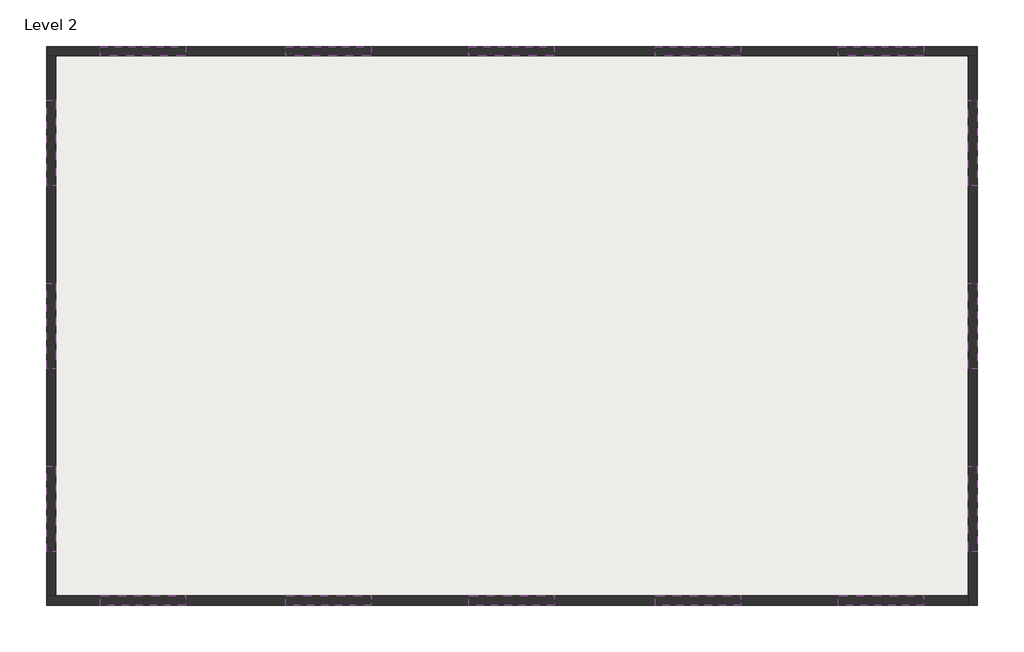
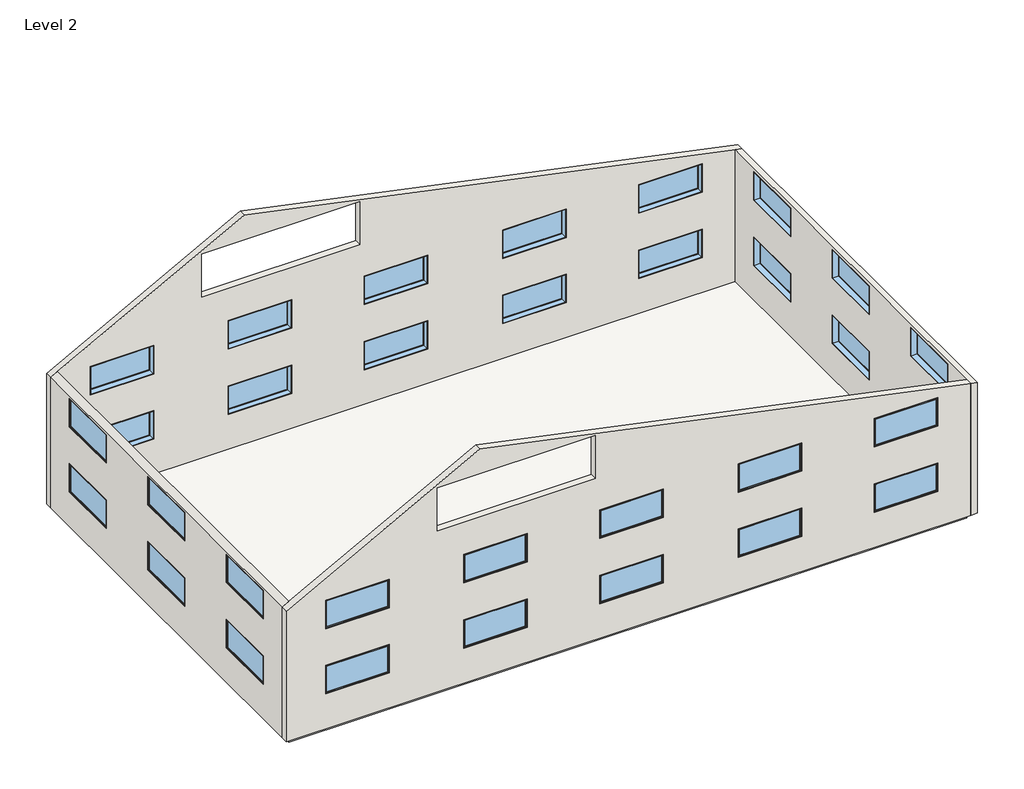
# One storey: 32 windows, 4 walls, 1 slab.
"""IFC4 building model written with IfcOpenShell, lengths in millimetres."""

import ifcopenshell
import ifcopenshell.guid

model = None  # the IFC model being written
_history = None  # IfcOwnerHistory: only IFC2X3 demands one
_inside = {}  # id of a spatial element -> (the spatial element, [elements in it])
_under = {}  # id of a project, library or spatial element -> (it, [spatial elements below it])
_declared = {}  # id of a project -> (the project, [libraries it declares])
_typed = {}  # id of a type object -> (the type object, [elements of that type])
_made_of = {}  # id of a material, layer set ... -> (it, [elements and type objects made of it])


def new_model(schema):
    """Start an empty IFC model of exactly this schema.

    Asked for "IFC4X3", IfcOpenShell would pick the latest addendum, in which some entities
    have other attributes; the version numbers below select the first issue.
    IFC2X3 requires an IfcOwnerHistory on every rooted entity: one is made here for all.
    """
    global model, _history
    if schema == "IFC4X3":
        model = ifcopenshell.file(schema_version=(4, 3, 0, 0))
    else:
        model = ifcopenshell.file(schema=schema)
    _inside.clear()
    _under.clear()
    _declared.clear()
    _typed.clear()
    _made_of.clear()
    _history = None
    if model.schema == "IFC2X3":
        org = make("IfcOrganization", Name="unknown")
        user = make(
            "IfcPersonAndOrganization",
            ThePerson=make("IfcPerson", FamilyName="unknown"),
            TheOrganization=org,
        )
        app = make(
            "IfcApplication",
            ApplicationDeveloper=org,
            Version="unknown",
            ApplicationFullName="unknown",
            ApplicationIdentifier="unknown",
        )
        _history = make(
            "IfcOwnerHistory",
            OwningUser=user,
            OwningApplication=app,
            ChangeAction="ADDED",
            CreationDate=0,
        )
    return model


def make(cls, **values):
    """One entity of the class cls with the attributes given. An attribute that is None is left unset."""
    return model.create_entity(
        cls, **{name: value for name, value in values.items() if value is not None}
    )


def rooted(cls, **values):
    """An entity with a GlobalId (a new one), such as an element, a storey or a relation."""
    return make(cls, GlobalId=ifcopenshell.guid.new(), OwnerHistory=_history, **values)


def si_unit(unit_type, name, prefix=None):
    """IfcSIUnit, for example si_unit("LENGTHUNIT", "METRE", prefix="MILLI")."""
    return make("IfcSIUnit", UnitType=unit_type, Prefix=prefix, Name=name)


def assignment(units):
    """IfcUnitAssignment: the units of a project."""
    return None if units is None else make("IfcUnitAssignment", Units=units)


def point(xyz):
    """IfcCartesianPoint."""
    return None if xyz is None else make("IfcCartesianPoint", Coordinates=xyz)


def direction(xyz):
    """IfcDirection."""
    return None if xyz is None else make("IfcDirection", DirectionRatios=xyz)


def frame(location, z_axis=None, x_axis=None):
    """IfcAxis2Placement3D, a coordinate frame: its origin and axes. An axis left out is left unset."""
    return make(
        "IfcAxis2Placement3D",
        Location=point(location),
        Axis=direction(z_axis),
        RefDirection=direction(x_axis),
    )


def origin():
    """The frame at (0, 0, 0) with its axes left unset."""
    return frame((0.0, 0.0, 0.0))


def place(relative_to, where):
    """IfcLocalPlacement: puts the frame where relative to a parent placement (None: the world)."""
    return make(
        "IfcLocalPlacement", PlacementRelTo=relative_to, RelativePlacement=where
    )


def context(
    kind, dimensions, precision=None, world=None, true_north=None, identifier=None
):
    """IfcGeometricRepresentationContext, for example the 3D "Model" context."""
    return make(
        "IfcGeometricRepresentationContext",
        ContextIdentifier=identifier,
        ContextType=kind,
        CoordinateSpaceDimension=dimensions,
        Precision=precision,
        WorldCoordinateSystem=world,
        TrueNorth=true_north,
    )


def project(units=None, contexts=None):
    """IfcProject with its units and contexts."""
    return rooted(
        "IfcProject",
        Name="project",
        RepresentationContexts=contexts,
        UnitsInContext=assignment(units),
    )


def spatial(cls, under=None, at=None, **own):
    """A site, building, storey or space (cls), placed at a placement, below another one or the project."""
    s = rooted(cls, ObjectPlacement=at, **own)
    if under is not None:
        _under.setdefault(under.id(), (under, []))[1].append(s)
    return s


def polyline(points):
    """IfcPolyline through the points."""
    return make("IfcPolyline", Points=[point(p) for p in points])


def outline(outer, holes=None, kind="AREA"):
    """IfcArbitraryClosedProfileDef: a profile drawn as a closed curve; with holes, ...WithVoids."""
    if holes is None:
        return make("IfcArbitraryClosedProfileDef", ProfileType=kind, OuterCurve=outer)
    return make(
        "IfcArbitraryProfileDefWithVoids",
        ProfileType=kind,
        OuterCurve=outer,
        InnerCurves=holes,
    )


def extrude(swept, where, along, depth):
    """IfcExtrudedAreaSolid: the profile swept, set in the frame where, extruded along a direction by depth."""
    return make(
        "IfcExtrudedAreaSolid",
        SweptArea=swept,
        Position=where,
        ExtrudedDirection=direction(along),
        Depth=depth,
    )


def faces_of(points, faces, orient=None, outer=None):
    """IfcFace entities. A face is a list of loops; a loop is a list of indices into points, from 0.

    orient and outer hold one flag for each loop. By default every Orientation is true, the
    first loop of a face is its IfcFaceOuterBound and the others are IfcFaceBound.
    """
    made = []
    for i, loops in enumerate(faces):
        bounds = []
        for j, loop in enumerate(loops):
            is_outer = j == 0 if outer is None else outer[i][j]
            bounds.append(
                make(
                    "IfcFaceOuterBound" if is_outer else "IfcFaceBound",
                    Bound=make("IfcPolyLoop", Polygon=[points[k] for k in loop]),
                    Orientation=True if orient is None else orient[i][j],
                )
            )
        made.append(make("IfcFace", Bounds=bounds))
    return made


def faceted_brep(points, faces, orient=None, outer=None, voids=None):
    """IfcFacetedBrep: a solid bounded by flat faces; with voids (closed shells), ...WithVoids."""
    shared = [point(p) for p in points]
    hull = make("IfcClosedShell", CfsFaces=faces_of(shared, faces, orient, outer))
    if voids is None:
        return make("IfcFacetedBrep", Outer=hull)
    return make(
        "IfcFacetedBrepWithVoids",
        Outer=hull,
        Voids=[
            make(cls, CfsFaces=faces_of(shared, fs, o, b)) for cls, fs, o, b in voids
        ],
    )


def shape(context_of_items, identifier, shape_type, items):
    """IfcShapeRepresentation: the items that make up one representation, for example the "Body"."""
    return make(
        "IfcShapeRepresentation",
        ContextOfItems=context_of_items,
        RepresentationIdentifier=identifier,
        RepresentationType=shape_type,
        Items=items,
    )


def source(mapping_origin, context_of_items, identifier, shape_type, items):
    """IfcRepresentationMap: a shape defined once, which mapped items show again and again."""
    return make(
        "IfcRepresentationMap",
        MappingOrigin=mapping_origin,
        MappedRepresentation=shape(context_of_items, identifier, shape_type, items),
    )


def transform(
    local_origin,
    x_axis=None,
    y_axis=None,
    z_axis=None,
    scale=None,
    scale2=None,
    scale3=None,
    uniform=True,
):
    """IfcCartesianTransformationOperator3D, or its non-uniform kind. x_axis, y_axis, z_axis: its Axis1, 2, 3."""
    if uniform:
        return make(
            "IfcCartesianTransformationOperator3D",
            Axis1=direction(x_axis),
            Axis2=direction(y_axis),
            LocalOrigin=point(local_origin),
            Scale=scale,
            Axis3=direction(z_axis),
        )
    return make(
        "IfcCartesianTransformationOperator3DnonUniform",
        Axis1=direction(x_axis),
        Axis2=direction(y_axis),
        LocalOrigin=point(local_origin),
        Scale=scale,
        Axis3=direction(z_axis),
        Scale2=scale2,
        Scale3=scale3,
    )


def mapped(mapping_source, mapping_target):
    """IfcMappedItem: shows the shape of a source again, moved by a transform."""
    return make(
        "IfcMappedItem", MappingSource=mapping_source, MappingTarget=mapping_target
    )


def made_of(thing, what):
    """Note that an element or type object is made of a material, layer set ...; save() writes the relation."""
    if what is not None:
        _made_of.setdefault(what.id(), (what, []))[1].append(thing)
    return thing


def element(
    cls,
    number,
    at=None,
    inside=None,
    cuts=None,
    type_object=None,
    material=None,
    context=None,
    identifier="Body",
    shape_type=None,
    held_by="IfcProductDefinitionShape",
    body=None,
    shapes=None,
    **own,
):
    """One element of the class cls, such as IfcWall. Its Tag is "e" and its number.

    at: its placement. inside: the storey or other place that contains it. cuts: it is an
    opening in that element (IfcRelVoidsElement). A single representation is given by context,
    identifier, shape_type and body (its items); several are given by shapes. held_by: the class
    of the entity that holds the representations. save() writes the other relations.
    """
    e = rooted(cls, Tag="e%d" % number, ObjectPlacement=at, **own)
    if body is not None:
        shapes = [shape(context, identifier, shape_type, body)]
    if shapes is not None:
        e.Representation = make(held_by, Representations=shapes)
    if inside is not None:
        _inside.setdefault(inside.id(), (inside, []))[1].append(e)
    if cuts is not None:
        rooted(
            "IfcRelVoidsElement", RelatingBuildingElement=cuts, RelatedOpeningElement=e
        )
    if type_object is not None:
        _typed.setdefault(type_object.id(), (type_object, []))[1].append(e)
    return made_of(e, material)


def aggregate(whole, parts):
    """IfcRelAggregates: a whole, such as a stair, and the parts it consists of."""
    return rooted("IfcRelAggregates", RelatingObject=whole, RelatedObjects=parts)


def save(model, path):
    """Write the relations noted so far, then the file.

    IfcRelAggregates (storeys below a building ...), IfcRelContainedInSpatialStructure (elements
    in a storey), IfcRelDefinesByType, IfcRelAssociatesMaterial and IfcRelDeclares: one each for
    every whole, place, type object, material and project.
    """
    for whole, parts in _under.values():
        aggregate(whole, parts)
    for where, things in _inside.values():
        rooted(
            "IfcRelContainedInSpatialStructure",
            RelatedElements=things,
            RelatingStructure=where,
        )
    for kind, things in _typed.values():
        rooted("IfcRelDefinesByType", RelatedObjects=things, RelatingType=kind)
    for what, things in _made_of.values():
        rooted("IfcRelAssociatesMaterial", RelatedObjects=things, RelatingMaterial=what)
    for by, libraries in _declared.values():
        rooted("IfcRelDeclares", RelatingContext=by, RelatedDefinitions=libraries)
    model.write(path)


def m_fixed_2800x_1327mm_376a1ccb(model_context):
    return source(origin(), model_context, "Body", "SweptSolid", [
        extrude(outline(polyline([(-1337.0, 130.4), (1337.0, 130.4), (1337.0, 118.4), (-1337.0, 118.4), (-1337.0, 130.4)])), frame((0.0, 0.0, 978.0), z_axis=(0.0, 0.0, 1.0), x_axis=(1.0, 0.0, 0.0)), (0.0, 0.0, 1.0), 1201.2),
        extrude(outline(polyline([(2223.2, -1381.0), (934.0, -1381.0), (934.0, 1381.0), (2223.2, 1381.0), (2223.2, -1381.0)]), holes=[polyline([(2179.2, -1337.0), (2179.2, 1337.0), (978.0, 1337.0), (978.0, -1337.0), (2179.2, -1337.0)])]), frame((0.0, 102.4, 0.0), z_axis=(0.0, 1.0, 0.0), x_axis=(0.0, 0.0, 1.0)), (0.0, 0.0, 1.0), 44.0),
        extrude(outline(polyline([(2242.2, -1400.0), (915.0, -1400.0), (915.0, 1400.0), (2242.2, 1400.0), (2242.2, -1400.0)]), holes=[polyline([(2223.2, -1381.0), (2223.2, 1381.0), (934.0, 1381.0), (934.0, -1381.0), (2223.2, -1381.0)])]), frame((0.0, 102.4, 0.0), z_axis=(0.0, 1.0, 0.0), x_axis=(0.0, 0.0, 1.0)), (0.0, 0.0, 1.0), 63.0),
        extrude(outline(polyline([(2242.2, -1400.0), (915.0, -1400.0), (915.0, 1400.0), (2242.2, 1400.0), (2242.2, -1400.0)]), holes=[polyline([(2210.2, -1368.0), (2210.2, 1368.0), (947.0, 1368.0), (947.0, -1368.0), (2210.2, -1368.0)])]), frame((0.0, -139.4, 0.0), z_axis=(0.0, 1.0, 0.0), x_axis=(0.0, 0.0, 1.0)), (0.0, 0.0, 1.0), 241.8),
    ])


def m_fixed_2800x_1327mm_95955449(model_context):
    return source(origin(), model_context, "Body", "SweptSolid", [
        extrude(outline(polyline([(-1337.0, -130.4), (-1337.0, -118.4), (1337.0, -118.4), (1337.0, -130.4), (-1337.0, -130.4)])), frame((0.0, 0.0, 978.0), z_axis=(0.0, 0.0, 1.0), x_axis=(1.0, 0.0, 0.0)), (0.0, 0.0, 1.0), 1201.2),
        extrude(outline(polyline([(2223.2, -1381.0), (934.0, -1381.0), (934.0, 1381.0), (2223.2, 1381.0), (2223.2, -1381.0)]), holes=[polyline([(2179.2, -1337.0), (2179.2, 1337.0), (978.0, 1337.0), (978.0, -1337.0), (2179.2, -1337.0)])]), frame((0.0, -146.4, 0.0), z_axis=(0.0, 1.0, 0.0), x_axis=(0.0, 0.0, 1.0)), (0.0, 0.0, 1.0), 44.0),
        extrude(outline(polyline([(2242.2, -1400.0), (915.0, -1400.0), (915.0, 1400.0), (2242.2, 1400.0), (2242.2, -1400.0)]), holes=[polyline([(2223.2, -1381.0), (2223.2, 1381.0), (934.0, 1381.0), (934.0, -1381.0), (2223.2, -1381.0)])]), frame((0.0, -165.4, 0.0), z_axis=(0.0, 1.0, 0.0), x_axis=(0.0, 0.0, 1.0)), (0.0, 0.0, 1.0), 63.0),
        extrude(outline(polyline([(2242.2, -1400.0), (915.0, -1400.0), (915.0, 1400.0), (2242.2, 1400.0), (2242.2, -1400.0)]), holes=[polyline([(2210.2, -1368.0), (2210.2, 1368.0), (947.0, 1368.0), (947.0, -1368.0), (2210.2, -1368.0)])]), frame((0.0, -102.4, 0.0), z_axis=(0.0, 1.0, 0.0), x_axis=(0.0, 0.0, 1.0)), (0.0, 0.0, 1.0), 241.8),
    ])


model = new_model("IFC4")

# Units and contexts
model_context = context("Model", 3, world=origin())
ifc_project = project(units=[si_unit("LENGTHUNIT", "METRE", prefix="MILLI")], contexts=[model_context])

# Site, building, storey
site = spatial("IfcSite", under=ifc_project)
building = spatial("IfcBuilding", under=site)
storey = spatial("IfcBuildingStorey", under=building, Name="Level 2", Elevation=3048.0)

# Slab
placement = place(None, origin())
element("IfcSlab", 1, ObjectType="Generic Floor - 304.8mm", at=placement, inside=storey, context=model_context, shape_type="SweptSolid", body=[
    extrude(outline(polyline([(31352.2035739, 12078.5990339), (31352.2035739, -5599.8009661), (1481.8035739, -5599.8009661), (1481.8035739, 12078.5990339), (31352.2035739, 12078.5990339)])), frame((0.0, 0.0, 2743.2), z_axis=(0.0, 0.0, 1.0), x_axis=(1.0, 0.0, 0.0)), (0.0, 0.0, 1.0), 304.8),
])

# Walls
element("IfcWall", 2, ObjectType="Generic - 304.8mm", at=placement, inside=storey, context=model_context, shape_type="Brep", body=[
    faceted_brep([(1177.0035739, 12078.5990339, 3048.0), (1481.8035739, 12078.5990339, 3048.0), (31352.2035739, 12078.5990339, 3048.0), (31657.0035739, 12078.5990339, 3048.0), (31657.0035739, 12078.5990339, 9144.0), (31352.2035739, 12078.5990339, 9207.5), (9711.4035739, 12078.5990339, 13716.0), (1481.8035739, 12078.5990339, 9307.2857143), (1177.0035739, 12078.5990339, 9144.0), (15004.6035739, 12078.5990339, 4643.0), (15004.6035739, 12078.5990339, 5970.2), (17804.6035739, 12078.5990339, 5970.2), (17804.6035739, 12078.5990339, 4643.0), (2929.4035739, 12078.5990339, 4666.9423249), (2929.4035739, 12078.5990339, 5994.1423249), (5729.4035739, 12078.5990339, 5994.1423249), (5729.4035739, 12078.5990339, 4666.9423249), (9004.6035739, 12078.5990339, 4666.9423249), (9004.6035739, 12078.5990339, 5994.1423249), (11804.6035739, 12078.5990339, 5994.1423249), (11804.6035739, 12078.5990339, 4666.9423249), (21104.6035739, 12078.5990339, 4666.9423249), (21104.6035739, 12078.5990339, 5994.1423249), (23904.6035739, 12078.5990339, 5994.1423249), (23904.6035739, 12078.5990339, 4666.9423249), (27104.6035739, 12078.5990339, 4666.9423249), (27104.6035739, 12078.5990339, 5994.1423249), (29904.6035739, 12078.5990339, 5994.1423249), (29904.6035739, 12078.5990339, 4666.9423249), (15004.6035739, 12078.5990339, 7691.0), (15004.6035739, 12078.5990339, 9018.2), (17804.6035739, 12078.5990339, 9018.2), (17804.6035739, 12078.5990339, 7691.0), (2929.4035739, 12078.5990339, 7714.9423249), (2929.4035739, 12078.5990339, 9042.1423249), (5729.4035739, 12078.5990339, 9042.1423249), (5729.4035739, 12078.5990339, 7714.9423249), (9004.6035739, 12078.5990339, 7714.9423249), (9004.6035739, 12078.5990339, 9042.1423249), (11804.6035739, 12078.5990339, 9042.1423249), (11804.6035739, 12078.5990339, 7714.9423249), (21104.6035739, 12078.5990339, 7714.9423249), (21104.6035739, 12078.5990339, 9042.1423249), (23904.6035739, 12078.5990339, 9042.1423249), (23904.6035739, 12078.5990339, 7714.9423249), (27104.6035739, 12078.5990339, 7714.9423249), (27104.6035739, 12078.5990339, 9042.1423249), (29904.6035739, 12078.5990339, 9042.1423249), (29904.6035739, 12078.5990339, 7714.9423249), (7845.5535739, 12078.5990339, 10559.0), (7845.5535739, 12078.5990339, 12559.0), (14813.2535739, 12078.5990339, 12559.0), (14813.2535739, 12078.5990339, 10559.0), (1177.0035739, 12383.3990339, 3048.0), (1177.0035739, 12383.3990339, 9144.0), (9711.4035739, 12383.3990339, 13716.0), (31657.0035739, 12383.3990339, 9144.0), (31657.0035739, 12383.3990339, 3048.0), (15004.6035739, 12383.3990339, 4643.0), (17804.6035739, 12383.3990339, 4643.0), (17804.6035739, 12383.3990339, 5970.2), (15004.6035739, 12383.3990339, 5970.2), (2929.4035739, 12383.3990339, 4666.9423249), (5729.4035739, 12383.3990339, 4666.9423249), (5729.4035739, 12383.3990339, 5994.1423249), (2929.4035739, 12383.3990339, 5994.1423249), (9004.6035739, 12383.3990339, 4666.9423249), (11804.6035739, 12383.3990339, 4666.9423249), (11804.6035739, 12383.3990339, 5994.1423249), (9004.6035739, 12383.3990339, 5994.1423249), (21104.6035739, 12383.3990339, 4666.9423249), (23904.6035739, 12383.3990339, 4666.9423249), (23904.6035739, 12383.3990339, 5994.1423249), (21104.6035739, 12383.3990339, 5994.1423249), (27104.6035739, 12383.3990339, 4666.9423249), (29904.6035739, 12383.3990339, 4666.9423249), (29904.6035739, 12383.3990339, 5994.1423249), (27104.6035739, 12383.3990339, 5994.1423249), (15004.6035739, 12383.3990339, 7691.0), (17804.6035739, 12383.3990339, 7691.0), (17804.6035739, 12383.3990339, 9018.2), (15004.6035739, 12383.3990339, 9018.2), (2929.4035739, 12383.3990339, 7714.9423249), (5729.4035739, 12383.3990339, 7714.9423249), (5729.4035739, 12383.3990339, 9042.1423249), (2929.4035739, 12383.3990339, 9042.1423249), (9004.6035739, 12383.3990339, 7714.9423249), (11804.6035739, 12383.3990339, 7714.9423249), (11804.6035739, 12383.3990339, 9042.1423249), (9004.6035739, 12383.3990339, 9042.1423249), (21104.6035739, 12383.3990339, 7714.9423249), (23904.6035739, 12383.3990339, 7714.9423249), (23904.6035739, 12383.3990339, 9042.1423249), (21104.6035739, 12383.3990339, 9042.1423249), (27104.6035739, 12383.3990339, 7714.9423249), (29904.6035739, 12383.3990339, 7714.9423249), (29904.6035739, 12383.3990339, 9042.1423249), (27104.6035739, 12383.3990339, 9042.1423249), (7845.5535739, 12383.3990339, 10559.0), (14813.2535739, 12383.3990339, 10559.0), (14813.2535739, 12383.3990339, 12559.0), (7845.5535739, 12383.3990339, 12559.0)], [[[0, 1, 2, 3, 4, 5, 6, 7, 8], [9, 10, 11, 12], [13, 14, 15, 16], [17, 18, 19, 20], [21, 22, 23, 24], [25, 26, 27, 28], [29, 30, 31, 32], [33, 34, 35, 36], [37, 38, 39, 40], [41, 42, 43, 44], [45, 46, 47, 48], [49, 50, 51, 52]], [[53, 54, 55, 56, 57], [58, 59, 60, 61], [62, 63, 64, 65], [66, 67, 68, 69], [70, 71, 72, 73], [74, 75, 76, 77], [78, 79, 80, 81], [82, 83, 84, 85], [86, 87, 88, 89], [90, 91, 92, 93], [94, 95, 96, 97], [98, 99, 100, 101]], [[3, 2, 1, 0, 53, 57]], [[4, 3, 57, 56]], [[0, 8, 54, 53]], [[8, 7, 6, 55, 54]], [[6, 5, 4, 56, 55]], [[10, 9, 58, 61]], [[11, 10, 61, 60]], [[12, 11, 60, 59]], [[9, 12, 59, 58]], [[14, 13, 62, 65]], [[15, 14, 65, 64]], [[16, 15, 64, 63]], [[13, 16, 63, 62]], [[18, 17, 66, 69]], [[19, 18, 69, 68]], [[20, 19, 68, 67]], [[17, 20, 67, 66]], [[22, 21, 70, 73]], [[23, 22, 73, 72]], [[24, 23, 72, 71]], [[21, 24, 71, 70]], [[26, 25, 74, 77]], [[27, 26, 77, 76]], [[28, 27, 76, 75]], [[25, 28, 75, 74]], [[30, 29, 78, 81]], [[31, 30, 81, 80]], [[32, 31, 80, 79]], [[29, 32, 79, 78]], [[34, 33, 82, 85]], [[35, 34, 85, 84]], [[36, 35, 84, 83]], [[33, 36, 83, 82]], [[38, 37, 86, 89]], [[39, 38, 89, 88]], [[40, 39, 88, 87]], [[37, 40, 87, 86]], [[42, 41, 90, 93]], [[43, 42, 93, 92]], [[44, 43, 92, 91]], [[41, 44, 91, 90]], [[46, 45, 94, 97]], [[47, 46, 97, 96]], [[48, 47, 96, 95]], [[45, 48, 95, 94]], [[50, 49, 98, 101]], [[51, 50, 101, 100]], [[52, 51, 100, 99]], [[49, 52, 99, 98]]]),
])
element("IfcWall", 3, ObjectType="Generic - 304.8mm", at=placement, inside=storey, context=model_context, shape_type="Brep", body=[
    faceted_brep([(31352.2035739, 12078.5990339, 3048.0), (31352.2035739, -5599.8009661, 3048.0), (31352.2035739, -5904.6009661, 3048.0), (31352.2035739, -5904.6009661, 9207.5), (31352.2035739, -5599.8009661, 9207.5), (31352.2035739, 12078.5990339, 9207.5), (31352.2035739, -4152.2009661, 4666.9), (31352.2035739, -1352.2009661, 4666.9), (31352.2035739, -1352.2009661, 5994.1), (31352.2035739, -4152.2009661, 5994.1), (31352.2035739, 7830.9990339, 4666.9), (31352.2035739, 10630.9990339, 4666.9), (31352.2035739, 10630.9990339, 5994.1), (31352.2035739, 7830.9990339, 5994.1), (31352.2035739, 1839.3990339, 4666.9), (31352.2035739, 4639.3990339, 4666.9), (31352.2035739, 4639.3990339, 5994.1), (31352.2035739, 1839.3990339, 5994.1), (31352.2035739, -4152.2009661, 7714.9), (31352.2035739, -1352.2009661, 7714.9), (31352.2035739, -1352.2009661, 9042.1), (31352.2035739, -4152.2009661, 9042.1), (31352.2035739, 7830.9990339, 7714.9), (31352.2035739, 10630.9990339, 7714.9), (31352.2035739, 10630.9990339, 9042.1), (31352.2035739, 7830.9990339, 9042.1), (31352.2035739, 1839.3990339, 7714.9), (31352.2035739, 4639.3990339, 7714.9), (31352.2035739, 4639.3990339, 9042.1), (31352.2035739, 1839.3990339, 9042.1), (31657.0035739, 12078.5990339, 3048.0), (31657.0035739, 12078.5990339, 9144.0), (31657.0035739, -5904.6009661, 9144.0), (31657.0035739, -5904.6009661, 3048.0), (31657.0035739, -4152.2009661, 4666.9), (31657.0035739, -4152.2009661, 5994.1), (31657.0035739, -1352.2009661, 5994.1), (31657.0035739, -1352.2009661, 4666.9), (31657.0035739, 7830.9990339, 4666.9), (31657.0035739, 7830.9990339, 5994.1), (31657.0035739, 10630.9990339, 5994.1), (31657.0035739, 10630.9990339, 4666.9), (31657.0035739, 1839.3990339, 4666.9), (31657.0035739, 1839.3990339, 5994.1), (31657.0035739, 4639.3990339, 5994.1), (31657.0035739, 4639.3990339, 4666.9), (31657.0035739, -4152.2009661, 7714.9), (31657.0035739, -4152.2009661, 9042.1), (31657.0035739, -1352.2009661, 9042.1), (31657.0035739, -1352.2009661, 7714.9), (31657.0035739, 7830.9990339, 7714.9), (31657.0035739, 7830.9990339, 9042.1), (31657.0035739, 10630.9990339, 9042.1), (31657.0035739, 10630.9990339, 7714.9), (31657.0035739, 1839.3990339, 7714.9), (31657.0035739, 1839.3990339, 9042.1), (31657.0035739, 4639.3990339, 9042.1), (31657.0035739, 4639.3990339, 7714.9)], [[[0, 1, 2, 3, 4, 5], [6, 7, 8, 9], [10, 11, 12, 13], [14, 15, 16, 17], [18, 19, 20, 21], [22, 23, 24, 25], [26, 27, 28, 29]], [[30, 31, 32, 33], [34, 35, 36, 37], [38, 39, 40, 41], [42, 43, 44, 45], [46, 47, 48, 49], [50, 51, 52, 53], [54, 55, 56, 57]], [[2, 1, 0, 30, 33]], [[0, 5, 31, 30]], [[3, 2, 33, 32]], [[35, 34, 6, 9]], [[36, 35, 9, 8]], [[37, 36, 8, 7]], [[34, 37, 7, 6]], [[39, 38, 10, 13]], [[40, 39, 13, 12]], [[41, 40, 12, 11]], [[38, 41, 11, 10]], [[43, 42, 14, 17]], [[44, 43, 17, 16]], [[45, 44, 16, 15]], [[42, 45, 15, 14]], [[47, 46, 18, 21]], [[48, 47, 21, 20]], [[49, 48, 20, 19]], [[46, 49, 19, 18]], [[51, 50, 22, 25]], [[52, 51, 25, 24]], [[53, 52, 24, 23]], [[50, 53, 23, 22]], [[55, 54, 26, 29]], [[56, 55, 29, 28]], [[57, 56, 28, 27]], [[54, 57, 27, 26]], [[5, 4, 3, 32, 31]]]),
])
element("IfcWall", 4, ObjectType="Generic - 304.8mm", at=placement, inside=storey, context=model_context, shape_type="Brep", body=[
    faceted_brep([(31352.2035739, -5599.8009661, 3048.0), (1481.8035739, -5599.8009661, 3048.0), (1177.0035739, -5599.8009661, 3048.0), (1177.0035739, -5599.8009661, 9144.0), (1481.8035739, -5599.8009661, 9307.2857143), (9711.4035739, -5599.8009661, 13716.0), (31352.2035739, -5599.8009661, 9207.5), (15004.6035739, -5599.8009661, 4643.0), (17804.6035739, -5599.8009661, 4643.0), (17804.6035739, -5599.8009661, 5970.2), (15004.6035739, -5599.8009661, 5970.2), (2929.4035739, -5599.8009661, 4666.9423249), (5729.4035739, -5599.8009661, 4666.9423249), (5729.4035739, -5599.8009661, 5994.1423249), (2929.4035739, -5599.8009661, 5994.1423249), (9004.6035739, -5599.8009661, 4666.9423249), (11804.6035739, -5599.8009661, 4666.9423249), (11804.6035739, -5599.8009661, 5994.1423249), (9004.6035739, -5599.8009661, 5994.1423249), (21104.6035739, -5599.8009661, 4666.9423249), (23904.6035739, -5599.8009661, 4666.9423249), (23904.6035739, -5599.8009661, 5994.1423249), (21104.6035739, -5599.8009661, 5994.1423249), (27104.6035739, -5599.8009661, 4666.9423249), (29904.6035739, -5599.8009661, 4666.9423249), (29904.6035739, -5599.8009661, 5994.1423249), (27104.6035739, -5599.8009661, 5994.1423249), (15004.6035739, -5599.8009661, 7691.0), (17804.6035739, -5599.8009661, 7691.0), (17804.6035739, -5599.8009661, 9018.2), (15004.6035739, -5599.8009661, 9018.2), (2929.4035739, -5599.8009661, 7714.9423249), (5729.4035739, -5599.8009661, 7714.9423249), (5729.4035739, -5599.8009661, 9042.1423249), (2929.4035739, -5599.8009661, 9042.1423249), (9004.6035739, -5599.8009661, 7714.9423249), (11804.6035739, -5599.8009661, 7714.9423249), (11804.6035739, -5599.8009661, 9042.1423249), (9004.6035739, -5599.8009661, 9042.1423249), (21104.6035739, -5599.8009661, 7714.9423249), (23904.6035739, -5599.8009661, 7714.9423249), (23904.6035739, -5599.8009661, 9042.1423249), (21104.6035739, -5599.8009661, 9042.1423249), (27104.6035739, -5599.8009661, 7714.9423249), (29904.6035739, -5599.8009661, 7714.9423249), (29904.6035739, -5599.8009661, 9042.1423249), (27104.6035739, -5599.8009661, 9042.1423249), (7845.5535739, -5599.8009661, 10559.0), (14813.2535739, -5599.8009661, 10559.0), (14813.2535739, -5599.8009661, 12559.0), (7845.5535739, -5599.8009661, 12559.0), (31352.2035739, -5904.6009661, 3048.0), (31352.2035739, -5904.6009661, 9207.5), (9711.4035739, -5904.6009661, 13716.0), (1177.0035739, -5904.6009661, 9144.0), (1177.0035739, -5904.6009661, 3048.0), (15004.6035739, -5904.6009661, 4643.0), (15004.6035739, -5904.6009661, 5970.2), (17804.6035739, -5904.6009661, 5970.2), (17804.6035739, -5904.6009661, 4643.0), (2929.4035739, -5904.6009661, 4666.9423249), (2929.4035739, -5904.6009661, 5994.1423249), (5729.4035739, -5904.6009661, 5994.1423249), (5729.4035739, -5904.6009661, 4666.9423249), (9004.6035739, -5904.6009661, 4666.9423249), (9004.6035739, -5904.6009661, 5994.1423249), (11804.6035739, -5904.6009661, 5994.1423249), (11804.6035739, -5904.6009661, 4666.9423249), (21104.6035739, -5904.6009661, 4666.9423249), (21104.6035739, -5904.6009661, 5994.1423249), (23904.6035739, -5904.6009661, 5994.1423249), (23904.6035739, -5904.6009661, 4666.9423249), (27104.6035739, -5904.6009661, 4666.9423249), (27104.6035739, -5904.6009661, 5994.1423249), (29904.6035739, -5904.6009661, 5994.1423249), (29904.6035739, -5904.6009661, 4666.9423249), (15004.6035739, -5904.6009661, 7691.0), (15004.6035739, -5904.6009661, 9018.2), (17804.6035739, -5904.6009661, 9018.2), (17804.6035739, -5904.6009661, 7691.0), (2929.4035739, -5904.6009661, 7714.9423249), (2929.4035739, -5904.6009661, 9042.1423249), (5729.4035739, -5904.6009661, 9042.1423249), (5729.4035739, -5904.6009661, 7714.9423249), (9004.6035739, -5904.6009661, 7714.9423249), (9004.6035739, -5904.6009661, 9042.1423249), (11804.6035739, -5904.6009661, 9042.1423249), (11804.6035739, -5904.6009661, 7714.9423249), (21104.6035739, -5904.6009661, 7714.9423249), (21104.6035739, -5904.6009661, 9042.1423249), (23904.6035739, -5904.6009661, 9042.1423249), (23904.6035739, -5904.6009661, 7714.9423249), (27104.6035739, -5904.6009661, 7714.9423249), (27104.6035739, -5904.6009661, 9042.1423249), (29904.6035739, -5904.6009661, 9042.1423249), (29904.6035739, -5904.6009661, 7714.9423249), (7845.5535739, -5904.6009661, 10559.0), (7845.5535739, -5904.6009661, 12559.0), (14813.2535739, -5904.6009661, 12559.0), (14813.2535739, -5904.6009661, 10559.0)], [[[0, 1, 2, 3, 4, 5, 6], [7, 8, 9, 10], [11, 12, 13, 14], [15, 16, 17, 18], [19, 20, 21, 22], [23, 24, 25, 26], [27, 28, 29, 30], [31, 32, 33, 34], [35, 36, 37, 38], [39, 40, 41, 42], [43, 44, 45, 46], [47, 48, 49, 50]], [[51, 52, 53, 54, 55], [56, 57, 58, 59], [60, 61, 62, 63], [64, 65, 66, 67], [68, 69, 70, 71], [72, 73, 74, 75], [76, 77, 78, 79], [80, 81, 82, 83], [84, 85, 86, 87], [88, 89, 90, 91], [92, 93, 94, 95], [96, 97, 98, 99]], [[2, 1, 0, 51, 55]], [[0, 6, 52, 51]], [[3, 2, 55, 54]], [[6, 5, 53, 52]], [[5, 4, 3, 54, 53]], [[57, 56, 7, 10]], [[58, 57, 10, 9]], [[59, 58, 9, 8]], [[56, 59, 8, 7]], [[61, 60, 11, 14]], [[62, 61, 14, 13]], [[63, 62, 13, 12]], [[60, 63, 12, 11]], [[65, 64, 15, 18]], [[66, 65, 18, 17]], [[67, 66, 17, 16]], [[64, 67, 16, 15]], [[69, 68, 19, 22]], [[70, 69, 22, 21]], [[71, 70, 21, 20]], [[68, 71, 20, 19]], [[73, 72, 23, 26]], [[74, 73, 26, 25]], [[75, 74, 25, 24]], [[72, 75, 24, 23]], [[77, 76, 27, 30]], [[78, 77, 30, 29]], [[79, 78, 29, 28]], [[76, 79, 28, 27]], [[81, 80, 31, 34]], [[82, 81, 34, 33]], [[83, 82, 33, 32]], [[80, 83, 32, 31]], [[85, 84, 35, 38]], [[86, 85, 38, 37]], [[87, 86, 37, 36]], [[84, 87, 36, 35]], [[89, 88, 39, 42]], [[90, 89, 42, 41]], [[91, 90, 41, 40]], [[88, 91, 40, 39]], [[93, 92, 43, 46]], [[94, 93, 46, 45]], [[95, 94, 45, 44]], [[92, 95, 44, 43]], [[97, 96, 47, 50]], [[98, 97, 50, 49]], [[99, 98, 49, 48]], [[96, 99, 48, 47]]]),
])
element("IfcWall", 5, ObjectType="Generic - 304.8mm", at=placement, inside=storey, context=model_context, shape_type="Brep", body=[
    faceted_brep([(1481.8035739, -5599.8009661, 3048.0), (1481.8035739, 12078.5990339, 3048.0), (1481.8035739, 12078.5990339, 9307.2857143), (1481.8035739, -5599.8009661, 9307.2857143), (1481.8035739, -4152.2009661, 4666.9), (1481.8035739, -4152.2009661, 5994.1), (1481.8035739, -1352.2009661, 5994.1), (1481.8035739, -1352.2009661, 4666.9), (1481.8035739, 7830.9990339, 4666.9), (1481.8035739, 7830.9990339, 5994.1), (1481.8035739, 10630.9990339, 5994.1), (1481.8035739, 10630.9990339, 4666.9), (1481.8035739, 1839.3990339, 4666.9), (1481.8035739, 1839.3990339, 5994.1), (1481.8035739, 4639.3990339, 5994.1), (1481.8035739, 4639.3990339, 4666.9), (1481.8035739, -4152.2009661, 7714.9), (1481.8035739, -4152.2009661, 9042.1), (1481.8035739, -1352.2009661, 9042.1), (1481.8035739, -1352.2009661, 7714.9), (1481.8035739, 7830.9990339, 7714.9), (1481.8035739, 7830.9990339, 9042.1), (1481.8035739, 10630.9990339, 9042.1), (1481.8035739, 10630.9990339, 7714.9), (1481.8035739, 1839.3990339, 7714.9), (1481.8035739, 1839.3990339, 9042.1), (1481.8035739, 4639.3990339, 9042.1), (1481.8035739, 4639.3990339, 7714.9), (1177.0035739, -5599.8009661, 3048.0), (1177.0035739, -5599.8009661, 9144.0), (1177.0035739, 12078.5990339, 9144.0), (1177.0035739, 12078.5990339, 3048.0), (1177.0035739, -4152.2009661, 4666.9), (1177.0035739, -1352.2009661, 4666.9), (1177.0035739, -1352.2009661, 5994.1), (1177.0035739, -4152.2009661, 5994.1), (1177.0035739, 7830.9990339, 4666.9), (1177.0035739, 10630.9990339, 4666.9), (1177.0035739, 10630.9990339, 5994.1), (1177.0035739, 7830.9990339, 5994.1), (1177.0035739, 1839.3990339, 4666.9), (1177.0035739, 4639.3990339, 4666.9), (1177.0035739, 4639.3990339, 5994.1), (1177.0035739, 1839.3990339, 5994.1), (1177.0035739, -4152.2009661, 7714.9), (1177.0035739, -1352.2009661, 7714.9), (1177.0035739, -1352.2009661, 9042.1), (1177.0035739, -4152.2009661, 9042.1), (1177.0035739, 7830.9990339, 7714.9), (1177.0035739, 10630.9990339, 7714.9), (1177.0035739, 10630.9990339, 9042.1), (1177.0035739, 7830.9990339, 9042.1), (1177.0035739, 1839.3990339, 7714.9), (1177.0035739, 4639.3990339, 7714.9), (1177.0035739, 4639.3990339, 9042.1), (1177.0035739, 1839.3990339, 9042.1)], [[[0, 1, 2, 3], [4, 5, 6, 7], [8, 9, 10, 11], [12, 13, 14, 15], [16, 17, 18, 19], [20, 21, 22, 23], [24, 25, 26, 27]], [[28, 29, 30, 31], [32, 33, 34, 35], [36, 37, 38, 39], [40, 41, 42, 43], [44, 45, 46, 47], [48, 49, 50, 51], [52, 53, 54, 55]], [[1, 0, 28, 31]], [[0, 3, 29, 28]], [[2, 1, 31, 30]], [[5, 4, 32, 35]], [[6, 5, 35, 34]], [[7, 6, 34, 33]], [[4, 7, 33, 32]], [[9, 8, 36, 39]], [[10, 9, 39, 38]], [[11, 10, 38, 37]], [[8, 11, 37, 36]], [[13, 12, 40, 43]], [[14, 13, 43, 42]], [[15, 14, 42, 41]], [[12, 15, 41, 40]], [[17, 16, 44, 47]], [[18, 17, 47, 46]], [[19, 18, 46, 45]], [[16, 19, 45, 44]], [[21, 20, 48, 51]], [[22, 21, 51, 50]], [[23, 22, 50, 49]], [[20, 23, 49, 48]], [[25, 24, 52, 55]], [[26, 25, 55, 54]], [[27, 26, 54, 53]], [[24, 27, 53, 52]], [[3, 2, 30, 29]]]),
])

# Windows
m_fixed_2800x_1327mm_shape = m_fixed_2800x_1327mm_376a1ccb(model_context)
element("IfcWindow", 6, ObjectType="M_Fixed : 2800x 1327mm", at=placement, inside=storey, context=model_context, shape_type="MappedRepresentation", body=[
    mapped(m_fixed_2800x_1327mm_shape, transform((28504.6035739, 12217.9990339, 3751.9423249), x_axis=(1.0, 0.0, 0.0), y_axis=(0.0, 1.0, 0.0), z_axis=(0.0, 0.0, 1.0))),
])
element("IfcWindow", 7, ObjectType="M_Fixed : 2800x 1327mm", at=placement, inside=storey, context=model_context, shape_type="MappedRepresentation", body=[
    mapped(m_fixed_2800x_1327mm_shape, transform((22504.6035739, 12217.9990339, 3751.9423249), x_axis=(1.0, 0.0, 0.0), y_axis=(0.0, 1.0, 0.0), z_axis=(0.0, 0.0, 1.0))),
])
element("IfcWindow", 8, ObjectType="M_Fixed : 2800x 1327mm", at=placement, inside=storey, context=model_context, shape_type="MappedRepresentation", body=[
    mapped(m_fixed_2800x_1327mm_shape, transform((10404.6035739, 12217.9990339, 3751.9423249), x_axis=(1.0, 0.0, 0.0), y_axis=(0.0, 1.0, 0.0), z_axis=(0.0, 0.0, 1.0))),
])
element("IfcWindow", 9, ObjectType="M_Fixed : 2800x 1327mm", at=placement, inside=storey, context=model_context, shape_type="MappedRepresentation", body=[
    mapped(m_fixed_2800x_1327mm_shape, transform((4329.4035739, 12217.9990339, 3751.9423249), x_axis=(1.0, 0.0, 0.0), y_axis=(0.0, 1.0, 0.0), z_axis=(0.0, 0.0, 1.0))),
])
element("IfcWindow", 10, ObjectType="M_Fixed : 2800x 1327mm", at=placement, inside=storey, context=model_context, shape_type="MappedRepresentation", body=[
    mapped(m_fixed_2800x_1327mm_shape, transform((16404.6035739, 12217.9990339, 3728.0), x_axis=(1.0, 0.0, 0.0), y_axis=(0.0, 1.0, 0.0), z_axis=(0.0, 0.0, 1.0))),
])
element("IfcWindow", 11, ObjectType="M_Fixed : 2800x 1327mm", at=placement, inside=storey, context=model_context, shape_type="MappedRepresentation", body=[
    mapped(m_fixed_2800x_1327mm_shape, transform((28504.6035739, 12217.9990339, 6799.9423249), x_axis=(1.0, 0.0, 0.0), y_axis=(0.0, 1.0, 0.0), z_axis=(0.0, 0.0, 1.0))),
])
element("IfcWindow", 12, ObjectType="M_Fixed : 2800x 1327mm", at=placement, inside=storey, context=model_context, shape_type="MappedRepresentation", body=[
    mapped(m_fixed_2800x_1327mm_shape, transform((22504.6035739, 12217.9990339, 6799.9423249), x_axis=(1.0, 0.0, 0.0), y_axis=(0.0, 1.0, 0.0), z_axis=(0.0, 0.0, 1.0))),
])
element("IfcWindow", 13, ObjectType="M_Fixed : 2800x 1327mm", at=placement, inside=storey, context=model_context, shape_type="MappedRepresentation", body=[
    mapped(m_fixed_2800x_1327mm_shape, transform((10404.6035739, 12217.9990339, 6799.9423249), x_axis=(1.0, 0.0, 0.0), y_axis=(0.0, 1.0, 0.0), z_axis=(0.0, 0.0, 1.0))),
])
element("IfcWindow", 14, ObjectType="M_Fixed : 2800x 1327mm", at=placement, inside=storey, context=model_context, shape_type="MappedRepresentation", body=[
    mapped(m_fixed_2800x_1327mm_shape, transform((4329.4035739, 12217.9990339, 6799.9423249), x_axis=(1.0, 0.0, 0.0), y_axis=(0.0, 1.0, 0.0), z_axis=(0.0, 0.0, 1.0))),
])
element("IfcWindow", 15, ObjectType="M_Fixed : 2800x 1327mm", at=placement, inside=storey, context=model_context, shape_type="MappedRepresentation", body=[
    mapped(m_fixed_2800x_1327mm_shape, transform((16404.6035739, 12217.9990339, 6776.0), x_axis=(1.0, 0.0, 0.0), y_axis=(0.0, 1.0, 0.0), z_axis=(0.0, 0.0, 1.0))),
])
element("IfcWindow", 16, ObjectType="M_Fixed : 2800x 1327mm", at=placement, inside=storey, context=model_context, shape_type="MappedRepresentation", body=[
    mapped(m_fixed_2800x_1327mm_shape, transform((1342.4035739, 3239.3990339, 3751.9), x_axis=(0.0, 1.0, 0.0), y_axis=(-1.0, 0.0, 0.0), z_axis=(0.0, 0.0, 1.0))),
])
element("IfcWindow", 17, ObjectType="M_Fixed : 2800x 1327mm", at=placement, inside=storey, context=model_context, shape_type="MappedRepresentation", body=[
    mapped(m_fixed_2800x_1327mm_shape, transform((1342.4035739, 9230.9990339, 3751.9), x_axis=(0.0, 1.0, 0.0), y_axis=(-1.0, 0.0, 0.0), z_axis=(0.0, 0.0, 1.0))),
])
element("IfcWindow", 18, ObjectType="M_Fixed : 2800x 1327mm", at=placement, inside=storey, context=model_context, shape_type="MappedRepresentation", body=[
    mapped(m_fixed_2800x_1327mm_shape, transform((1342.4035739, -2752.2009661, 3751.9), x_axis=(0.0, 1.0, 0.0), y_axis=(-1.0, 0.0, 0.0), z_axis=(0.0, 0.0, 1.0))),
])
element("IfcWindow", 19, ObjectType="M_Fixed : 2800x 1327mm", at=placement, inside=storey, context=model_context, shape_type="MappedRepresentation", body=[
    mapped(m_fixed_2800x_1327mm_shape, transform((1342.4035739, 3239.3990339, 6799.9), x_axis=(0.0, 1.0, 0.0), y_axis=(-1.0, 0.0, 0.0), z_axis=(0.0, 0.0, 1.0))),
])
element("IfcWindow", 20, ObjectType="M_Fixed : 2800x 1327mm", at=placement, inside=storey, context=model_context, shape_type="MappedRepresentation", body=[
    mapped(m_fixed_2800x_1327mm_shape, transform((1342.4035739, 9230.9990339, 6799.9), x_axis=(0.0, 1.0, 0.0), y_axis=(-1.0, 0.0, 0.0), z_axis=(0.0, 0.0, 1.0))),
])
element("IfcWindow", 21, ObjectType="M_Fixed : 2800x 1327mm", at=placement, inside=storey, context=model_context, shape_type="MappedRepresentation", body=[
    mapped(m_fixed_2800x_1327mm_shape, transform((1342.4035739, -2752.2009661, 6799.9), x_axis=(0.0, 1.0, 0.0), y_axis=(-1.0, 0.0, 0.0), z_axis=(0.0, 0.0, 1.0))),
])
m_fixed_2800x_1327mm_2_shape = m_fixed_2800x_1327mm_95955449(model_context)
element("IfcWindow", 22, ObjectType="M_Fixed : 2800x 1327mm", at=placement, inside=storey, context=model_context, shape_type="MappedRepresentation", body=[
    mapped(m_fixed_2800x_1327mm_2_shape, transform((28504.6035739, -5739.2009661, 3751.9423249), x_axis=(1.0, 0.0, 0.0), y_axis=(0.0, 1.0, 0.0), z_axis=(0.0, 0.0, 1.0))),
])
element("IfcWindow", 23, ObjectType="M_Fixed : 2800x 1327mm", at=placement, inside=storey, context=model_context, shape_type="MappedRepresentation", body=[
    mapped(m_fixed_2800x_1327mm_2_shape, transform((22504.6035739, -5739.2009661, 3751.9423249), x_axis=(1.0, 0.0, 0.0), y_axis=(0.0, 1.0, 0.0), z_axis=(0.0, 0.0, 1.0))),
])
element("IfcWindow", 24, ObjectType="M_Fixed : 2800x 1327mm", at=placement, inside=storey, context=model_context, shape_type="MappedRepresentation", body=[
    mapped(m_fixed_2800x_1327mm_2_shape, transform((10404.6035739, -5739.2009661, 3751.9423249), x_axis=(1.0, 0.0, 0.0), y_axis=(0.0, 1.0, 0.0), z_axis=(0.0, 0.0, 1.0))),
])
element("IfcWindow", 25, ObjectType="M_Fixed : 2800x 1327mm", at=placement, inside=storey, context=model_context, shape_type="MappedRepresentation", body=[
    mapped(m_fixed_2800x_1327mm_2_shape, transform((4329.4035739, -5739.2009661, 3751.9423249), x_axis=(1.0, 0.0, 0.0), y_axis=(0.0, 1.0, 0.0), z_axis=(0.0, 0.0, 1.0))),
])
element("IfcWindow", 26, ObjectType="M_Fixed : 2800x 1327mm", at=placement, inside=storey, context=model_context, shape_type="MappedRepresentation", body=[
    mapped(m_fixed_2800x_1327mm_2_shape, transform((16404.6035739, -5739.2009661, 3728.0), x_axis=(1.0, 0.0, 0.0), y_axis=(0.0, 1.0, 0.0), z_axis=(0.0, 0.0, 1.0))),
])
element("IfcWindow", 27, ObjectType="M_Fixed : 2800x 1327mm", at=placement, inside=storey, context=model_context, shape_type="MappedRepresentation", body=[
    mapped(m_fixed_2800x_1327mm_2_shape, transform((28504.6035739, -5739.2009661, 6799.9423249), x_axis=(1.0, 0.0, 0.0), y_axis=(0.0, 1.0, 0.0), z_axis=(0.0, 0.0, 1.0))),
])
element("IfcWindow", 28, ObjectType="M_Fixed : 2800x 1327mm", at=placement, inside=storey, context=model_context, shape_type="MappedRepresentation", body=[
    mapped(m_fixed_2800x_1327mm_2_shape, transform((22504.6035739, -5739.2009661, 6799.9423249), x_axis=(1.0, 0.0, 0.0), y_axis=(0.0, 1.0, 0.0), z_axis=(0.0, 0.0, 1.0))),
])
element("IfcWindow", 29, ObjectType="M_Fixed : 2800x 1327mm", at=placement, inside=storey, context=model_context, shape_type="MappedRepresentation", body=[
    mapped(m_fixed_2800x_1327mm_2_shape, transform((10404.6035739, -5739.2009661, 6799.9423249), x_axis=(1.0, 0.0, 0.0), y_axis=(0.0, 1.0, 0.0), z_axis=(0.0, 0.0, 1.0))),
])
element("IfcWindow", 30, ObjectType="M_Fixed : 2800x 1327mm", at=placement, inside=storey, context=model_context, shape_type="MappedRepresentation", body=[
    mapped(m_fixed_2800x_1327mm_2_shape, transform((4329.4035739, -5739.2009661, 6799.9423249), x_axis=(1.0, 0.0, 0.0), y_axis=(0.0, 1.0, 0.0), z_axis=(0.0, 0.0, 1.0))),
])
element("IfcWindow", 31, ObjectType="M_Fixed : 2800x 1327mm", at=placement, inside=storey, context=model_context, shape_type="MappedRepresentation", body=[
    mapped(m_fixed_2800x_1327mm_2_shape, transform((16404.6035739, -5739.2009661, 6776.0), x_axis=(1.0, 0.0, 0.0), y_axis=(0.0, 1.0, 0.0), z_axis=(0.0, 0.0, 1.0))),
])
element("IfcWindow", 32, ObjectType="M_Fixed : 2800x 1327mm", at=placement, inside=storey, context=model_context, shape_type="MappedRepresentation", body=[
    mapped(m_fixed_2800x_1327mm_2_shape, transform((31491.6035739, 3239.3990339, 3751.9), x_axis=(0.0, 1.0, 0.0), y_axis=(-1.0, 0.0, 0.0), z_axis=(0.0, 0.0, 1.0))),
])
element("IfcWindow", 33, ObjectType="M_Fixed : 2800x 1327mm", at=placement, inside=storey, context=model_context, shape_type="MappedRepresentation", body=[
    mapped(m_fixed_2800x_1327mm_2_shape, transform((31491.6035739, 9230.9990339, 3751.9), x_axis=(0.0, 1.0, 0.0), y_axis=(-1.0, 0.0, 0.0), z_axis=(0.0, 0.0, 1.0))),
])
element("IfcWindow", 34, ObjectType="M_Fixed : 2800x 1327mm", at=placement, inside=storey, context=model_context, shape_type="MappedRepresentation", body=[
    mapped(m_fixed_2800x_1327mm_2_shape, transform((31491.6035739, -2752.2009661, 3751.9), x_axis=(0.0, 1.0, 0.0), y_axis=(-1.0, 0.0, 0.0), z_axis=(0.0, 0.0, 1.0))),
])
element("IfcWindow", 35, ObjectType="M_Fixed : 2800x 1327mm", at=placement, inside=storey, context=model_context, shape_type="MappedRepresentation", body=[
    mapped(m_fixed_2800x_1327mm_2_shape, transform((31491.6035739, 3239.3990339, 6799.9), x_axis=(0.0, 1.0, 0.0), y_axis=(-1.0, 0.0, 0.0), z_axis=(0.0, 0.0, 1.0))),
])
element("IfcWindow", 36, ObjectType="M_Fixed : 2800x 1327mm", at=placement, inside=storey, context=model_context, shape_type="MappedRepresentation", body=[
    mapped(m_fixed_2800x_1327mm_2_shape, transform((31491.6035739, 9230.9990339, 6799.9), x_axis=(0.0, 1.0, 0.0), y_axis=(-1.0, 0.0, 0.0), z_axis=(0.0, 0.0, 1.0))),
])
element("IfcWindow", 37, ObjectType="M_Fixed : 2800x 1327mm", at=placement, inside=storey, context=model_context, shape_type="MappedRepresentation", body=[
    mapped(m_fixed_2800x_1327mm_2_shape, transform((31491.6035739, -2752.2009661, 6799.9), x_axis=(0.0, 1.0, 0.0), y_axis=(-1.0, 0.0, 0.0), z_axis=(0.0, 0.0, 1.0))),
])

save(model, "model.ifc")

# Revit data of these elements
# Type "Generic Floor - 304.8mm"
#   Function = 0
#   Layers, outside or top first: 304.8 mm no material (function 1)
# Type "Generic - 304.8mm"
#   Layers, outside or top first: 304.8 mm no material (function 1)
# Type "M_Fixed : 2800x 1327mm"
#   Type Mark = "46"
#   Height = 1327.2 mm
#   Default Sill Height = 915 mm
#   Width = 2800 mm
#   Window Inset = 19 mm
#   Frame Exterior Material = Sash
#   Frame Interior Material = Sash
#   Glass Pane Material = Glass
#   Sash = Sash
#   Wall Closure = (empty or 0)
# Element 1 (IfcSlab, "Generic Floor - 304.8mm")
#   Height Offset From Level = 0 mm
#   Phase Created = New Construction
#   Materials on its faces: "Default Floor"
# Elements 2, 3, 4, 5 (IfcWall, "Generic - 304.8mm")
#   Top Offset = 0 mm
#   Base Offset = 0 mm
#   wall height = 6096 mm
#   Phase Created = New Construction
#   Base Constraint = Level 2
#   Top Constraint = Roof level
#   Materials on its faces: "Default Wall"
# Element 6 (IfcWindow, "M_Fixed : 2800x 1327mm")
#   Mark = "44"
#   Phase Created = New Construction
#   Materials on its faces: "Sash", "Glass"
# Element 7 (IfcWindow, "M_Fixed : 2800x 1327mm")
#   Mark = "45"
#   Phase Created = New Construction
#   Materials on its faces: "Sash", "Glass"
# Element 8 (IfcWindow, "M_Fixed : 2800x 1327mm")
#   Mark = "46"
#   Phase Created = New Construction
#   Materials on its faces: "Sash", "Glass"
# Element 9 (IfcWindow, "M_Fixed : 2800x 1327mm")
#   Mark = "47"
#   Phase Created = New Construction
#   Materials on its faces: "Sash", "Glass"
# Element 10 (IfcWindow, "M_Fixed : 2800x 1327mm")
#   Mark = "48"
#   Phase Created = New Construction
#   Materials on its faces: "Sash", "Glass"
# Element 11 (IfcWindow, "M_Fixed : 2800x 1327mm")
#   Mark = "49"
#   Phase Created = New Construction
#   Materials on its faces: "Sash", "Glass"
# Element 12 (IfcWindow, "M_Fixed : 2800x 1327mm")
#   Mark = "50"
#   Phase Created = New Construction
#   Materials on its faces: "Sash", "Glass"
# Element 13 (IfcWindow, "M_Fixed : 2800x 1327mm")
#   Mark = "51"
#   Phase Created = New Construction
#   Materials on its faces: "Sash", "Glass"
# Element 14 (IfcWindow, "M_Fixed : 2800x 1327mm")
#   Mark = "52"
#   Phase Created = New Construction
#   Materials on its faces: "Sash", "Glass"
# Element 15 (IfcWindow, "M_Fixed : 2800x 1327mm")
#   Mark = "53"
#   Phase Created = New Construction
#   Materials on its faces: "Sash", "Glass"
# Element 16 (IfcWindow, "M_Fixed : 2800x 1327mm")
#   Mark = "72"
#   Phase Created = New Construction
#   Materials on its faces: "Sash", "Glass"
# Element 17 (IfcWindow, "M_Fixed : 2800x 1327mm")
#   Mark = "73"
#   Phase Created = New Construction
#   Materials on its faces: "Sash", "Glass"
# Element 18 (IfcWindow, "M_Fixed : 2800x 1327mm")
#   Mark = "74"
#   Phase Created = New Construction
#   Materials on its faces: "Sash", "Glass"
# Element 19 (IfcWindow, "M_Fixed : 2800x 1327mm")
#   Mark = "75"
#   Phase Created = New Construction
#   Materials on its faces: "Sash", "Glass"
# Element 20 (IfcWindow, "M_Fixed : 2800x 1327mm")
#   Mark = "76"
#   Phase Created = New Construction
#   Materials on its faces: "Sash", "Glass"
# Element 21 (IfcWindow, "M_Fixed : 2800x 1327mm")
#   Mark = "77"
#   Phase Created = New Construction
#   Materials on its faces: "Sash", "Glass"
# Element 22 (IfcWindow, "M_Fixed : 2800x 1327mm")
#   Mark = "59"
#   Phase Created = New Construction
#   Materials on its faces: "Sash", "Glass"
# Element 23 (IfcWindow, "M_Fixed : 2800x 1327mm")
#   Mark = "60"
#   Phase Created = New Construction
#   Materials on its faces: "Sash", "Glass"
# Element 24 (IfcWindow, "M_Fixed : 2800x 1327mm")
#   Mark = "61"
#   Phase Created = New Construction
#   Materials on its faces: "Sash", "Glass"
# Element 25 (IfcWindow, "M_Fixed : 2800x 1327mm")
#   Mark = "62"
#   Phase Created = New Construction
#   Materials on its faces: "Sash", "Glass"
# Element 26 (IfcWindow, "M_Fixed : 2800x 1327mm")
#   Mark = "63"
#   Phase Created = New Construction
#   Materials on its faces: "Sash", "Glass"
# Element 27 (IfcWindow, "M_Fixed : 2800x 1327mm")
#   Mark = "64"
#   Phase Created = New Construction
#   Materials on its faces: "Sash", "Glass"
# Element 28 (IfcWindow, "M_Fixed : 2800x 1327mm")
#   Mark = "65"
#   Phase Created = New Construction
#   Materials on its faces: "Sash", "Glass"
# Element 29 (IfcWindow, "M_Fixed : 2800x 1327mm")
#   Mark = "66"
#   Phase Created = New Construction
#   Materials on its faces: "Sash", "Glass"
# Element 30 (IfcWindow, "M_Fixed : 2800x 1327mm")
#   Mark = "67"
#   Phase Created = New Construction
#   Materials on its faces: "Sash", "Glass"
# Element 31 (IfcWindow, "M_Fixed : 2800x 1327mm")
#   Mark = "68"
#   Phase Created = New Construction
#   Materials on its faces: "Sash", "Glass"
# Element 32 (IfcWindow, "M_Fixed : 2800x 1327mm")
#   Mark = "81"
#   Phase Created = New Construction
#   Materials on its faces: "Sash", "Glass"
# Element 33 (IfcWindow, "M_Fixed : 2800x 1327mm")
#   Mark = "82"
#   Phase Created = New Construction
#   Materials on its faces: "Sash", "Glass"
# Element 34 (IfcWindow, "M_Fixed : 2800x 1327mm")
#   Mark = "83"
#   Phase Created = New Construction
#   Materials on its faces: "Sash", "Glass"
# Element 35 (IfcWindow, "M_Fixed : 2800x 1327mm")
#   Mark = "84"
#   Phase Created = New Construction
#   Materials on its faces: "Sash", "Glass"
# Element 36 (IfcWindow, "M_Fixed : 2800x 1327mm")
#   Mark = "85"
#   Phase Created = New Construction
#   Materials on its faces: "Sash", "Glass"
# Element 37 (IfcWindow, "M_Fixed : 2800x 1327mm")
#   Mark = "86"
#   Phase Created = New Construction
#   Materials on its faces: "Sash", "Glass"
# Materials
#   "Sash": class "Wood", colour RGB 136 99 55, transparency 0
#   "Glass": class "Glass", colour RGB 0 128 192, transparency 0.9, Description = "Soda Lime Glass", Cost = 0
#   "Default Floor": class "Miscellaneous", colour RGB 127 127 127, transparency 0, Cost = 0
#   "Default Wall": class "Miscellaneous", colour RGB 128 128 128, transparency 0, Cost = 0
# Room at (16236.864, 2368.195) mm, phase "New Construction", upper level "Top roof", upper offset 0 mm, lower offset 0 mm
#   Number = "2"
#   Name = "Room"
